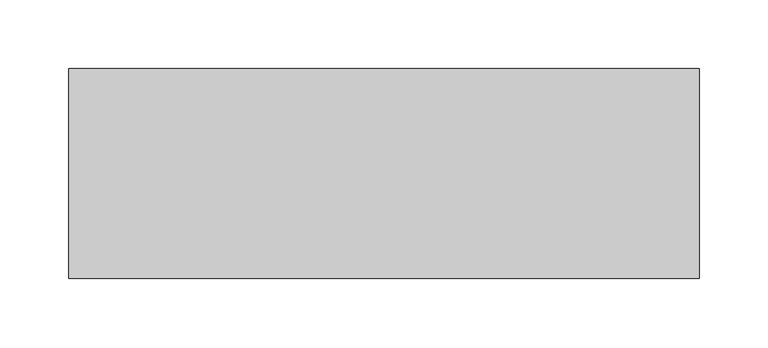
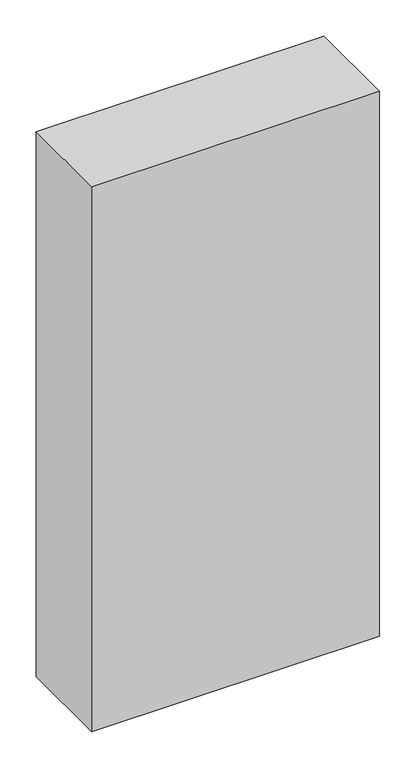
"""IFC4 building model written with IfcOpenShell, lengths in millimetres: proxy geometry, 262400 - Switchboards and Panelboards - Electric Panel - Generic : 262400 - Switchboards and Panelboards - Electric Panel - Generic."""

from ifc_helpers import new_model, si_unit, frame, origin, place, context, project, spatial, polyline, outline, extrude, source, transform, mapped, element, save


def electrical_equipment_ff41b5c6(model_context):
    return source(origin(), model_context, "Body", "SweptSolid", [
        extrude(outline(polyline([(457.2, 0.0), (0.0, 0.0), (0.0, 152.4), (457.2, 152.4), (457.2, 0.0)])), frame((0.0, 0.0, 457.2), z_axis=(0.0, 0.0, 1.0), x_axis=(1.0, 0.0, 0.0)), (0.0, 0.0, 1.0), 914.4),
    ])


if __name__ == "__main__":
    model = new_model("IFC4")
    model_context = context("Model", 3, world=origin())
    ifc_project = project(units=[si_unit("LENGTHUNIT", "METRE", prefix="MILLI")], contexts=[model_context])
    site = spatial("IfcSite", under=ifc_project)
    building = spatial("IfcBuilding", under=site)
    placement = place(None, origin())
    electrical_equipment_shape = electrical_equipment_ff41b5c6(model_context)
    element("IfcBuildingElementProxy", 1, Name="262400 - Switchboards and Panelboards - Electric Panel - Generic : 262400 - Switchboards and Panelboards - Electric Panel - Generic", ObjectType="262400 - Switchboards and Panelboards - Electric Panel - Generic : 262400 - Switchboards and Panelboards - Electric Panel - Generic", at=placement, inside=building, context=model_context, shape_type="MappedRepresentation", body=[
        mapped(electrical_equipment_shape, transform((0.0, 0.0, 0.0), x_axis=(1.0, 0.0, 0.0), y_axis=(0.0, 1.0, 0.0), z_axis=(0.0, 0.0, 1.0))),
    ])
    save(model, "model.ifc")

# Revit data of these elements
# Type "262400 - Switchboards and Panelboards - Electric Panel - Generic : 262400 - Switchboards and Panelboards - Electric Panel - Generic"
#   Width [instance default] = 1' - 6"
#   Off the Floor [instance default] = 1' - 6"
#   Height [instance default] = 3' - 0"
#   Depth [instance default] = 0' - 6"
#   Material = ELECTRICAL PANELS
# Element 1 (IfcBuildingElementProxy, "262400 - Switchboards and Panelboards - Electric Panel - Generic : 262400 - Switchboards and Panelboards - Electric Panel - Generic")
#   Materials on its faces: "ELECTRICAL PANELS"
# Materials
#   "ELECTRICAL PANELS": class "Generic", colour RGB 255 255 255, transparency 0, Cost = 0
